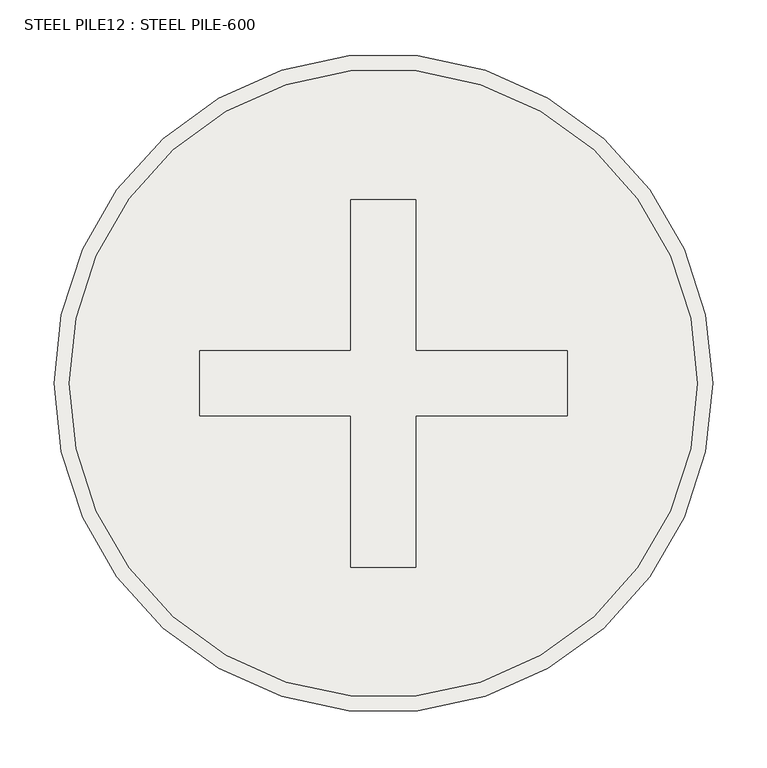
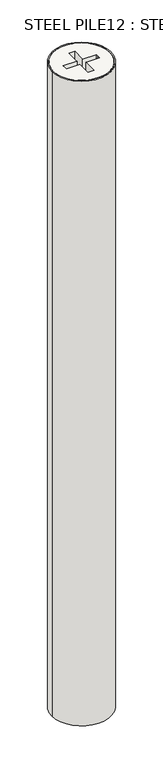
"""IFC4 building model written with IfcOpenShell, lengths in millimetres: slab geometry, STEEL PILE12 : STEEL PILE-600."""

from ifc_helpers import new_model, si_unit, point, frame, frame_2d, origin, place, context, project, spatial, circle_curve, trimmed, segment, composite_curve, outline, extrude, source, transform, mapped, element, save
from ifc_brep_helpers import plane_surface, cylinder_surface, advanced_brep


def steel_pile12_steel_pile_600_d6c65e66(model_context):
    return source(origin(), model_context, "Body", "SolidModel", [
        advanced_brep(
        [(8709.5, 19499.5208589, 150.0), (9290.5, 19499.5208589, 150.0), (8970.0, 19469.5208589, 150.0), (8830.0, 19469.5208589, 150.0), (8830.0, 19499.5208589, 150.0), (8830.0, 19529.5208589, 150.0), (8970.0, 19529.5208589, 150.0), (8970.0, 19669.5208589, 150.0), (9030.0, 19669.5208589, 150.0), (9030.0, 19529.5208589, 150.0), (9170.0, 19529.5208589, 150.0), (9170.0, 19499.5208589, 150.0), (9170.0, 19469.5208589, 150.0), (9030.0, 19469.5208589, 150.0), (9030.0, 19329.5208589, 150.0), (8970.0, 19329.5208589, 150.0), (8709.5, 19499.5208589, -1850.0), (9290.5, 19499.5208589, -1850.0), (8830.0, 19469.5208589, -160.0), (8970.0, 19469.5208589, -160.0), (8970.0, 19329.5208589, -160.0), (9030.0, 19329.5208589, -160.0), (9030.0, 19469.5208589, -160.0), (9170.0, 19469.5208589, -160.0), (9170.0, 19499.5208589, -160.0), (9170.0, 19529.5208589, -160.0), (9030.0, 19529.5208589, -160.0), (9030.0, 19669.5208589, -160.0), (8970.0, 19669.5208589, -160.0), (8970.0, 19529.5208589, -160.0), (8830.0, 19529.5208589, -160.0), (8830.0, 19499.5208589, -160.0)],
        [
            (0, 1, circle_curve(frame((9000.0, 19499.5208589, 150.0), z_axis=(0.0, 0.0, 1.0), x_axis=(1.0, 0.0, 0.0)), 290.5)),
            (1, 0, circle_curve(frame((9000.0, 19499.5208589, 150.0), z_axis=(0.0, 0.0, 1.0), x_axis=(1.0, 0.0, 0.0)), 290.5)),
            (2, 3),
            (3, 4),
            (4, 5),
            (5, 6),
            (6, 7),
            (7, 8),
            (8, 9),
            (9, 10),
            (10, 11),
            (11, 12),
            (12, 13),
            (13, 14),
            (14, 15),
            (15, 2),
            (16, 17, circle_curve(frame((9000.0, 19499.5208589, -1850.0), z_axis=(0.0, 0.0, -1.0), x_axis=(1.0, 0.0, 0.0)), 290.5)),
            (17, 16, circle_curve(frame((9000.0, 19499.5208589, -1850.0), z_axis=(0.0, 0.0, -1.0), x_axis=(1.0, 0.0, 0.0)), 290.5)),
            (0, 16),
            (17, 1),
            (18, 19),
            (19, 20),
            (20, 21),
            (21, 22),
            (22, 23),
            (23, 24),
            (24, 25),
            (25, 26),
            (26, 27),
            (27, 28),
            (28, 29),
            (29, 30),
            (30, 31),
            (31, 18),
            (18, 3),
            (2, 19),
            (15, 20),
            (14, 21),
            (13, 22),
            (12, 23),
            (11, 24),
            (10, 25),
            (9, 26),
            (8, 27),
            (7, 28),
            (6, 29),
            (5, 30),
            (4, 31),
        ],
        [
            plane_surface(frame((9290.5, 19499.5208589, 150.0), z_axis=(0.0, 0.0, 1.0), x_axis=(0.0, 1.0, 0.0))),
            plane_surface(frame((9290.5, 19499.5208589, -1850.0), z_axis=(0.0, 0.0, -1.0), x_axis=(0.0, -1.0, 0.0))),
            cylinder_surface(frame((9000.0, 19499.5208589, -1850.0), z_axis=(0.0, 0.0, 1.0), x_axis=(1.0, 0.0, 0.0)), 290.5),
            plane_surface(frame((8830.0, 19469.5208589, -160.0), z_axis=(0.0, 0.0, 1.0), x_axis=(-1.0, 0.0, 0.0))),
            plane_surface(frame((8830.0, 19469.5208589, 160.0), z_axis=(0.0, 1.0, 0.0), x_axis=(0.0, 0.0, -1.0))),
            plane_surface(frame((8970.0, 19469.5208589, 160.0), z_axis=(1.0, 0.0, 0.0), x_axis=(0.0, 0.0, -1.0))),
            plane_surface(frame((8970.0, 19329.5208589, 160.0), z_axis=(0.0, 1.0, 0.0), x_axis=(0.0, 0.0, -1.0))),
            plane_surface(frame((9030.0, 19329.5208589, 160.0), z_axis=(-1.0, 0.0, 0.0), x_axis=(0.0, 0.0, -1.0))),
            plane_surface(frame((9030.0, 19469.5208589, 160.0), z_axis=(0.0, 1.0, 0.0), x_axis=(0.0, 0.0, -1.0))),
            plane_surface(frame((9170.0, 19469.5208589, 160.0), z_axis=(-1.0, 0.0, 0.0), x_axis=(0.0, 0.0, -1.0))),
            plane_surface(frame((9170.0, 19499.5208589, 160.0), z_axis=(-1.0, 0.0, 0.0), x_axis=(0.0, 0.0, -1.0))),
            plane_surface(frame((9170.0, 19529.5208589, 160.0), z_axis=(0.0, -1.0, 0.0), x_axis=(0.0, 0.0, -1.0))),
            plane_surface(frame((9030.0, 19529.5208589, 160.0), z_axis=(-1.0, 0.0, 0.0), x_axis=(0.0, 0.0, -1.0))),
            plane_surface(frame((9030.0, 19669.5208589, 160.0), z_axis=(0.0, -1.0, 0.0), x_axis=(0.0, 0.0, -1.0))),
            plane_surface(frame((8970.0, 19669.5208589, 160.0), z_axis=(1.0, 0.0, 0.0), x_axis=(0.0, 0.0, -1.0))),
            plane_surface(frame((8970.0, 19529.5208589, 160.0), z_axis=(0.0, -1.0, 0.0), x_axis=(0.0, 0.0, -1.0))),
            plane_surface(frame((8830.0, 19529.5208589, 160.0), z_axis=(1.0, 0.0, 0.0), x_axis=(0.0, 0.0, -1.0))),
            plane_surface(frame((8830.0, 19499.5208589, 160.0), z_axis=(1.0, 0.0, 0.0), x_axis=(0.0, 0.0, -1.0))),
        ],
        [
            (0, [[1, 2], [3, 4, 5, 6, 7, 8, 9, 10, 11, 12, 13, 14, 15, 16]]),
            (1, [[17, 18]]),
            (2, [[-1, 19, -18, 20]]),
            (2, [[-2, -20, -17, -19]]),
            (3, [[21, 22, 23, 24, 25, 26, 27, 28, 29, 30, 31, 32, 33, 34]]),
            (4, [[-21, 35, -3, 36]]),
            (5, [[-22, -36, -16, 37]]),
            (6, [[-23, -37, -15, 38]]),
            (7, [[-24, -38, -14, 39]]),
            (8, [[-25, -39, -13, 40]]),
            (9, [[-26, -40, -12, 41]]),
            (10, [[-27, -41, -11, 42]]),
            (11, [[-28, -42, -10, 43]]),
            (12, [[-29, -43, -9, 44]]),
            (13, [[-30, -44, -8, 45]]),
            (14, [[-31, -45, -7, 46]]),
            (15, [[-32, -46, -6, 47]]),
            (16, [[-33, -47, -5, 48]]),
            (17, [[-34, -48, -4, -35]]),
        ],
    ),
        extrude(outline(composite_curve([segment(trimmed(circle_curve(frame_2d((9000.0, 19499.5208589)), 304.5), [point((8695.5, 19499.5208589))], [point((9304.5, 19499.5208589))], False, "CARTESIAN"), True, "CONTINUOUS"), segment(trimmed(circle_curve(frame_2d((9000.0, 19499.5208589)), 304.5), [point((9304.5, 19499.5208589))], [point((8695.5, 19499.5208589))], False, "CARTESIAN"), True, "CONTINUOUS")], self_intersect=False), holes=[composite_curve([segment(trimmed(circle_curve(frame_2d((9000.0, 19499.5208589)), 290.5), [point((8709.5, 19499.5208589))], [point((9290.5, 19499.5208589))], True, "CARTESIAN"), True, "CONTINUOUS"), segment(trimmed(circle_curve(frame_2d((9000.0, 19499.5208589)), 290.5), [point((9290.5, 19499.5208589))], [point((8709.5, 19499.5208589))], True, "CARTESIAN"), True, "CONTINUOUS")], self_intersect=False)]), frame((0.0, 0.0, -6850.0), z_axis=(0.0, 0.0, 1.0), x_axis=(1.0, 0.0, 0.0)), (0.0, 0.0, 1.0), 7000.0),
    ])


if __name__ == "__main__":
    model = new_model("IFC4")
    model_context = context("Model", 3, world=origin())
    ifc_project = project(units=[si_unit("LENGTHUNIT", "METRE", prefix="MILLI")], contexts=[model_context])
    site = spatial("IfcSite", under=ifc_project)
    building = spatial("IfcBuilding", under=site)
    placement = place(None, origin())
    steel_pile12_steel_pile_600_shape = steel_pile12_steel_pile_600_d6c65e66(model_context)
    element("IfcSlab", 1, ObjectType="STEEL PILE12 : STEEL PILE-600", at=placement, inside=building, context=model_context, shape_type="MappedRepresentation", body=[
        mapped(steel_pile12_steel_pile_600_shape, transform((0.0, 0.0, 0.0), x_axis=(1.0, 0.0, 0.0), y_axis=(0.0, 1.0, 0.0), z_axis=(0.0, 0.0, 1.0))),
    ])
    save(model, "model.ifc")
